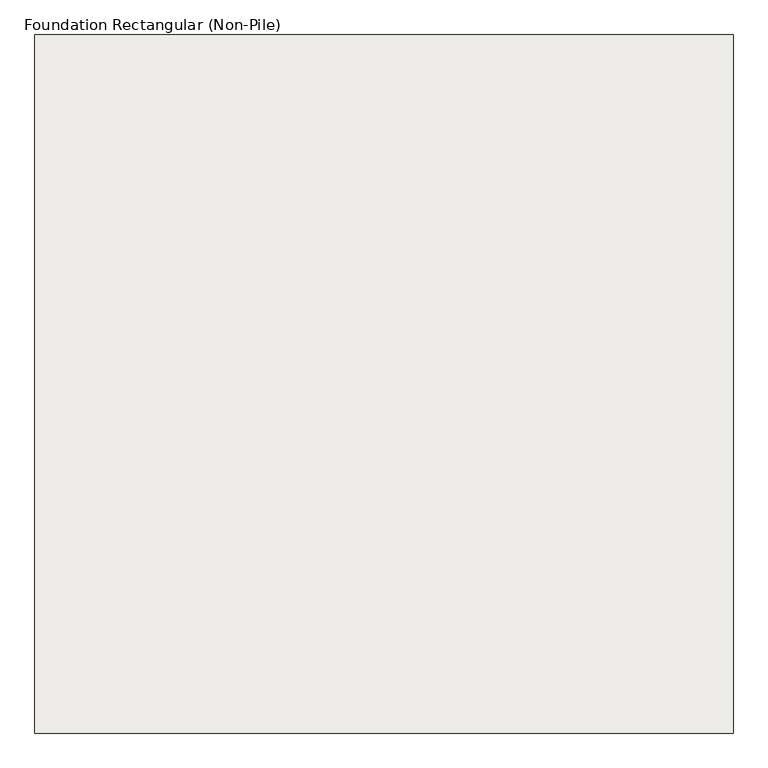
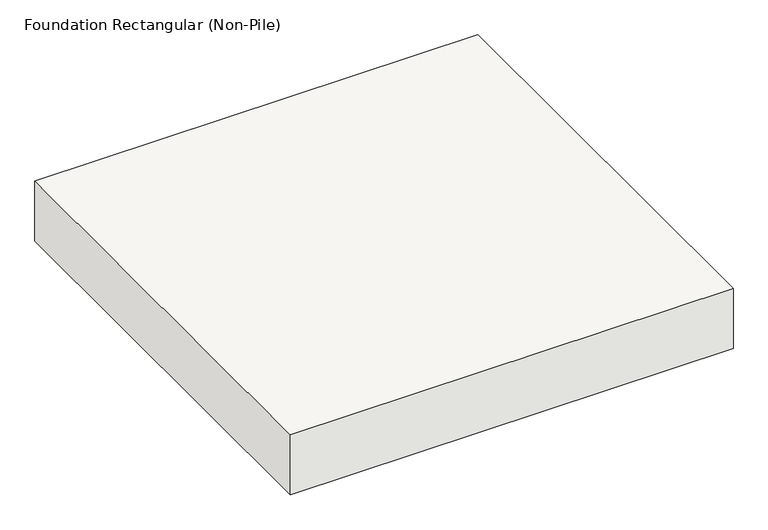
"""IFC4 building model written with IfcOpenShell, lengths in millimetres: slab geometry, Foundation Rectangular (Non-Pile) : H_SF_AR S18_Ret Fdn_F3 3500x3500x600."""

from ifc_helpers import new_model, si_unit, frame, origin, place, context, project, spatial, polyline, outline, extrude, source, transform, mapped, element, save


def foundation_rectangular_non_pile_20b31725(model_context):
    return source(origin(), model_context, "Body", "SweptSolid", [
        extrude(outline(polyline([(1750.0, 1750.0), (1750.0, -1750.0), (-1750.0, -1750.0), (-1750.0, 1750.0), (1750.0, 1750.0)])), frame((0.0, 0.0, -500.0), z_axis=(0.0, 0.0, 1.0), x_axis=(1.0, 0.0, 0.0)), (0.0, 0.0, 1.0), 500.0),
    ])


if __name__ == "__main__":
    model = new_model("IFC4")
    model_context = context("Model", 3, world=origin())
    ifc_project = project(units=[si_unit("LENGTHUNIT", "METRE", prefix="MILLI")], contexts=[model_context])
    site = spatial("IfcSite", under=ifc_project)
    building = spatial("IfcBuilding", under=site)
    placement = place(None, origin())
    foundation_rectangular_non_pile_shape = foundation_rectangular_non_pile_20b31725(model_context)
    element("IfcSlab", 1, ObjectType="Foundation Rectangular (Non-Pile) : H_SF_AR S18_Ret Fdn_F3 3500x3500x600", at=placement, inside=building, context=model_context, shape_type="MappedRepresentation", body=[
        mapped(foundation_rectangular_non_pile_shape, transform((0.0, 0.0, 0.0), x_axis=(1.0, 0.0, 0.0), y_axis=(0.0, 1.0, 0.0), z_axis=(0.0, 0.0, 1.0))),
    ])
    save(model, "model.ifc")

# Revit data of these elements
# Project information
#   H_Building Area = "0.00 m²"
#   H_Building H = "0"
#   H_Building L = "0"
#   H_Building NOS = "1"
#   H_Building Story = "1"
#   H_Building Total Area = "0.00 m²"
#   H_Building W = "0"
#   H_Building Volume = "0.000 m³"
#   H_Seismic Condition = "A as per ASCE 7-10"
#   H_Soil Condition = "C as per ASCE 7-10"
#   H_Basic Wind Speed = "58.3m/s ASCE7-10"
#   H_DS Project Code = "FAASA2302"
#   H_Project Abbreviation = "SACE2"
#   H_Project Division = "화공"
#   H_Project Finish = "2027-03-05"
#   H_Project Location = "Jafurah, Saudi Arabia"
#   H_Project Start = "2024-01-03"
#   H_Project Type = "EPC"
#   H_Smart Code = "FAASA2302"
#   Project Issue Date = "Issue Date"
#   Project Status = "Project Status"
#   Client Name = "Owner"
#   Project Address = "Enter address here"
#   Project Name = "Project Name"
#   Project Number = "0001"
# Type "Foundation Rectangular (Non-Pile) : H_SF_AR S18_Ret Fdn_F3 3500x3500x600"
#   Type Comments = "UG"
#   Type Mark = "F3"
#   Top bar = "D25@300"
#   Description = "UG Shallow Foundation"
#   Bottom bar = "D20@300"
#   H_Rebar Ratio = 0.12
#   Width = 3500 mm
#   Length = 3500 mm
#   Foundation Thickness = 500 mm
#   Structural Material [instance default] = none
#   Assembly Code = ""
# Element 1 (IfcSlab, "Foundation Rectangular (Non-Pile) : H_SF_AR S18_Ret Fdn_F3 3500x3500x600")
#   Materials on its faces: "00_Concrete_Reinf. Conc."
# Materials
#   "00_Concrete_Reinf. Conc.": class "Concrete", colour RGB 176 176 176, transparency 0, Description = "Reinf. Conc.", Cost = 0, Image = Concrete.Cast-In-Place.Flat.Polished.Grey.jpg
